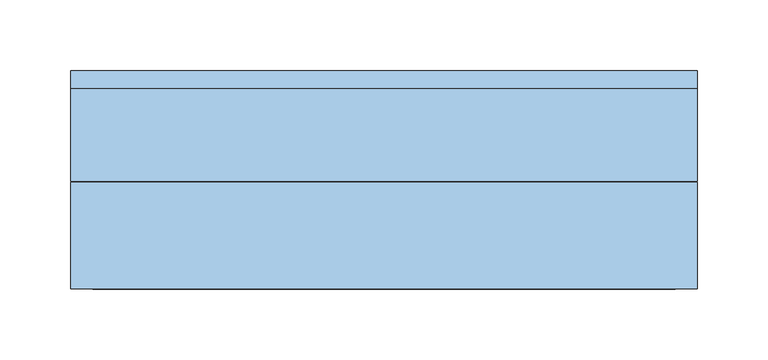
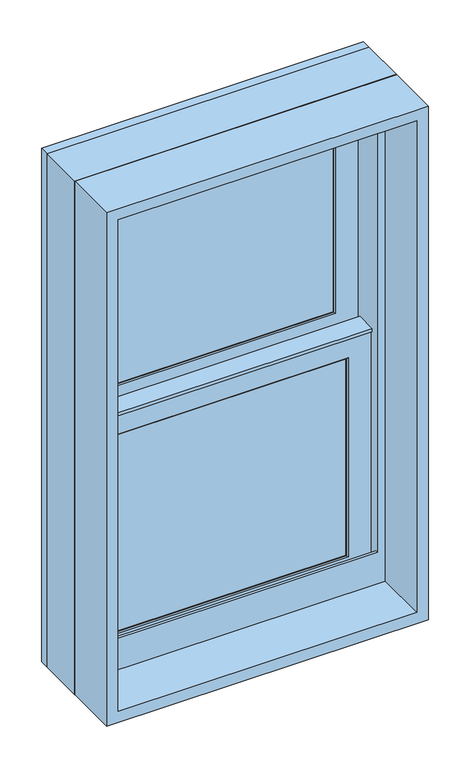
"""IFC4 building model written with IfcOpenShell, lengths in millimetres: window geometry, Window-Double_Hung-Marvin-Essential : ESDH1626."""

from ifc_helpers import new_model, si_unit, frame, origin, place, context, project, spatial, polyline, outline, extrude, faceted_brep, source, transform, mapped, element, save


def window_9d5250ab(model_context):
    return source(origin(), model_context, "Body", "SolidModel", [
        extrude(outline(polyline([(64.5583333, 20.6375), (64.5583333, 15.875), (45.5083333, 15.875), (45.5083333, 20.6375), (64.5583333, 20.6375)])), frame((0.0, 0.0, 1746.25), z_axis=(0.0, 0.0, 1.0), x_axis=(1.0, 0.0, 0.0)), (0.0, 0.0, 1.0), 298.45),
        extrude(outline(polyline([(-45.5083333, 20.6375), (-45.5083333, 15.875), (-64.5583333, 15.875), (-64.5583333, 20.6375), (-45.5083333, 20.6375)])), frame((0.0, 0.0, 1746.25), z_axis=(0.0, 0.0, 1.0), x_axis=(1.0, 0.0, 0.0)), (0.0, 0.0, 1.0), 298.45),
        extrude(outline(polyline([(165.1, 20.6375), (165.1, 15.875), (-165.1, 15.875), (-165.1, 20.6375), (165.1, 20.6375)])), frame((0.0, 0.0, 1885.95), z_axis=(0.0, 0.0, 1.0), x_axis=(1.0, 0.0, 0.0)), (0.0, 0.0, 1.0), 19.05),
        extrude(outline(polyline([(-64.5583333, 46.83125), (-64.5583333, 51.59375), (-45.5083333, 51.59375), (-45.5083333, 46.83125), (-64.5583333, 46.83125)])), frame((0.0, 0.0, 2082.8), z_axis=(0.0, 0.0, 1.0), x_axis=(1.0, 0.0, 0.0)), (0.0, 0.0, 1.0), 298.45),
        extrude(outline(polyline([(45.5083333, 46.83125), (45.5083333, 51.59375), (64.5583333, 51.59375), (64.5583333, 46.83125), (45.5083333, 46.83125)])), frame((0.0, 0.0, 2082.8), z_axis=(0.0, 0.0, 1.0), x_axis=(1.0, 0.0, 0.0)), (0.0, 0.0, 1.0), 298.45),
        extrude(outline(polyline([(-165.1, 46.83125), (-165.1, 51.59375), (165.1, 51.59375), (165.1, 46.83125), (-165.1, 46.83125)])), frame((0.0, 0.0, 2222.5), z_axis=(0.0, 0.0, 1.0), x_axis=(1.0, 0.0, 0.0)), (0.0, 0.0, 1.0), 19.05),
        extrude(outline(polyline([(64.5583333, 20.6375), (45.5083333, 20.6375), (45.5083333, 25.4), (64.5583333, 25.4), (64.5583333, 20.6375)])), frame((0.0, 0.0, 1746.25), z_axis=(0.0, 0.0, 1.0), x_axis=(1.0, 0.0, 0.0)), (0.0, 0.0, 1.0), 298.45),
        extrude(outline(polyline([(-45.5083333, 20.6375), (-64.5583333, 20.6375), (-64.5583333, 25.4), (-45.5083333, 25.4), (-45.5083333, 20.6375)])), frame((0.0, 0.0, 1746.25), z_axis=(0.0, 0.0, 1.0), x_axis=(1.0, 0.0, 0.0)), (0.0, 0.0, 1.0), 298.45),
        extrude(outline(polyline([(165.1, 20.6375), (-165.1, 20.6375), (-165.1, 25.4), (165.1, 25.4), (165.1, 20.6375)])), frame((0.0, 0.0, 1885.95), z_axis=(0.0, 0.0, 1.0), x_axis=(1.0, 0.0, 0.0)), (0.0, 0.0, 1.0), 19.05),
        extrude(outline(polyline([(-64.5583333, 56.35625), (-45.5083333, 56.35625), (-45.5083333, 51.59375), (-64.5583333, 51.59375), (-64.5583333, 56.35625)])), frame((0.0, 0.0, 2082.8), z_axis=(0.0, 0.0, 1.0), x_axis=(1.0, 0.0, 0.0)), (0.0, 0.0, 1.0), 298.45),
        extrude(outline(polyline([(45.5083333, 56.35625), (64.5583333, 56.35625), (64.5583333, 51.59375), (45.5083333, 51.59375), (45.5083333, 56.35625)])), frame((0.0, 0.0, 2082.8), z_axis=(0.0, 0.0, 1.0), x_axis=(1.0, 0.0, 0.0)), (0.0, 0.0, 1.0), 298.45),
        extrude(outline(polyline([(-165.1, 56.35625), (165.1, 56.35625), (165.1, 51.59375), (-165.1, 51.59375), (-165.1, 56.35625)])), frame((0.0, 0.0, 2222.5), z_axis=(0.0, 0.0, 1.0), x_axis=(1.0, 0.0, 0.0)), (0.0, 0.0, 1.0), 19.05),
        faceted_brep([(-192.0875, 5.6780605, 2074.7351748), (-192.0875, 5.6780605, 2070.1), (192.0875, 5.6780605, 2070.1), (192.0875, 5.6780605, 2074.7351748), (-192.0875, 34.8118605, 2074.7351748), (192.0875, 34.8118605, 2074.7351748), (192.0875, 34.8118605, 2070.1), (-192.0875, 34.8118605, 2070.1), (-192.0875, 30.1625, 2070.1), (-192.0875, 30.1625, 1719.2625), (-192.0875, 8.9241104, 1719.2625), (-192.0875, 8.9241104, 2070.1), (192.0875, 8.9241104, 2070.1), (192.0875, 30.1625, 2070.1), (192.0875, 8.9241104, 1719.2625), (192.0875, 30.1625, 1719.2625), (-176.2034752, 11.90625, 2055.8034752), (-176.2034752, 30.1625, 2055.8034752), (176.2034752, 30.1625, 2055.8034752), (176.2034752, 11.90625, 2055.8034752), (-159.54375, 10.4662439, 2039.14375), (-159.54375, 11.90625, 2039.14375), (159.54375, 11.90625, 2039.14375), (159.54375, 10.4662439, 2039.14375), (161.0858834, 8.9241104, 2040.6858834), (-161.0858834, 8.9241104, 2040.6858834), (176.2034752, 30.1625, 1735.1465248), (176.2034752, 11.90625, 1735.1465248), (159.54375, 11.90625, 1751.80625), (159.54375, 10.4662439, 1751.80625), (161.0858834, 8.9241104, 1750.2641166), (-176.2034752, 30.1625, 1735.1465248), (-176.2034752, 11.90625, 1735.1465248), (-159.54375, 11.90625, 1751.80625), (-159.54375, 10.4662439, 1751.80625), (-161.0858834, 8.9241104, 1750.2641166)], [[[0, 1, 2, 3]], [[4, 5, 6, 7]], [[1, 0, 4, 7, 8, 9, 10, 11]], [[2, 1, 11, 12]], [[7, 6, 13, 8]], [[3, 2, 12, 14, 15, 13, 6, 5]], [[0, 3, 5, 4]], [[16, 17, 18, 19]], [[20, 21, 22, 23]], [[20, 23, 24, 25]], [[19, 18, 26, 27]], [[23, 22, 28, 29]], [[24, 23, 29, 30]], [[27, 26, 31, 32]], [[29, 28, 33, 34]], [[30, 29, 34, 35]], [[15, 14, 10, 9]], [[15, 9, 8, 13], [18, 17, 31, 26]], [[17, 16, 32, 31]], [[16, 19, 27, 32], [22, 21, 33, 28]], [[21, 20, 34, 33]], [[20, 25, 35, 34]], [[10, 14, 12, 11], [25, 24, 30, 35]]]),
        extrude(outline(polyline([(38.5955581, 2055.8125), (33.5778968, 2055.8125), (33.5778968, 2057.4), (39.9405976, 2057.4), (39.9405976, 2055.8125), (61.515625, 2055.8125), (47.6307501, 2052.4975159), (38.5955581, 2052.4975159), (38.5955581, 2055.8125)])), frame((-192.0875, 0.0, 0.0), z_axis=(1.0, 0.0, 0.0), x_axis=(0.0, 1.0, 0.0)), (0.0, 0.0, 1.0), 384.175),
        faceted_brep([(222.25, 0.0, 1689.1), (222.25, 0.0, 2438.4), (-222.25, 0.0, 2438.4), (-222.25, 0.0, 1689.1), (196.05625, 0.0, 1750.21875), (-196.05625, 0.0, 1750.21875), (-196.05625, 0.0, 2412.20625), (196.05625, 0.0, 2412.20625), (196.05625, 3.96875, 1689.1), (-196.05625, 3.96875, 1689.1), (-196.05625, 3.96875, 1750.21875), (196.05625, 3.96875, 1750.21875), (-222.25, 65.6828125, 1689.1), (-196.05625, 65.6828125, 1689.1), (196.05625, 65.6828125, 1689.1), (222.25, 65.6828125, 1689.1), (-222.25, 65.6828125, 2438.4), (222.25, 65.6828125, 2438.4), (196.05625, 65.6828125, 2412.20625), (-196.05625, 65.6828125, 2412.20625)], [[[0, 1, 2, 3], [4, 5, 6, 7]], [[8, 9, 10, 11]], [[5, 4, 11, 10]], [[0, 3, 12, 13, 9, 8, 14, 15]], [[13, 12, 16, 17, 15, 14, 18, 19]], [[13, 19, 6, 5, 10, 9]], [[7, 6, 19, 18]], [[18, 14, 8, 11, 4, 7]], [[1, 0, 15, 17]], [[2, 1, 17, 16]], [[3, 2, 16, 12]]]),
        faceted_brep([(196.05625, 30.1625, 2063.75), (194.46875, 30.1625, 2063.75), (194.46875, 30.1625, 1713.4544613), (196.05625, 30.1625, 1713.4544613), (-194.46875, 30.1625, 2063.75), (-196.05625, 30.1625, 2063.75), (-196.05625, 30.1625, 1713.4544613), (-194.46875, 30.1625, 1713.4544613), (194.46875, 63.5, 2063.75), (196.05625, 63.5, 2063.75), (196.05625, 63.5, 1706.9743077), (194.46875, 63.5, 1706.9743077), (-196.05625, 63.5, 2063.75), (-194.46875, 63.5, 2063.75), (-194.46875, 63.5, 1706.9743077), (-196.05625, 63.5, 1706.9743077), (207.3108932, 3.96875, 1718.5460105), (207.3108932, 3.96875, 1689.1), (207.3108932, 65.6828125, 1689.1), (207.3108932, 65.6828125, 1706.550012), (-207.3108932, 3.96875, 1689.1), (-207.3108932, 3.96875, 1718.5460105), (-207.3108932, 65.6828125, 1706.550012), (-207.3108932, 65.6828125, 1689.1), (207.3108932, 78.58125, 1704.0428097), (-207.3108932, 78.58125, 1704.0428097), (-205.2971252, 68.2348864, 1706.0539391), (-187.33135, 68.2348864, 1706.0539391), (-187.33135, 65.6828125, 1706.550012), (187.33135, 65.6828125, 1706.550012), (187.33135, 68.2348864, 1706.0539391), (205.2971252, 68.2348864, 1706.0539391), (-222.25, 65.6828125, 1689.1), (-222.25, 78.5948249, 1689.1), (222.25, 78.5948249, 1689.1), (222.25, 65.6828125, 1689.1), (-222.25, 78.58125, 2438.4), (222.25, 78.58125, 2438.4), (207.3108932, 78.58125, 2423.4608932), (-207.3108932, 78.58125, 2423.4608932), (-222.25, 65.6828125, 2438.4), (-205.2971252, 68.2348864, 2421.4471252), (205.2971252, 68.2348864, 2421.4471252), (187.33135, 68.2348864, 2403.48135), (-187.33135, 68.2348864, 2403.48135), (-187.33135, 65.6828125, 2403.48135), (187.33135, 65.6828125, 2403.48135), (222.25, 65.6828125, 2438.4)], [[[0, 1, 2, 3]], [[4, 5, 6, 7]], [[8, 9, 10, 11]], [[12, 13, 14, 15]], [[1, 8, 11, 2]], [[9, 0, 3, 10]], [[1, 0, 9, 8]], [[5, 4, 13, 12]], [[5, 12, 15, 6]], [[13, 4, 7, 14]], [[16, 17, 18, 19]], [[20, 21, 22, 23]], [[24, 25, 26, 27, 28, 22, 21, 16, 19, 29, 30, 31], [3, 2, 11, 10], [7, 6, 15, 14]], [[17, 16, 21, 20]], [[17, 20, 23, 32, 33, 34, 35, 18]], [[34, 33, 36, 37], [25, 24, 38, 39]], [[33, 32, 40, 36]], [[39, 41, 26, 25]], [[41, 42, 31, 30, 43, 44, 27, 26]], [[44, 45, 28, 27]], [[40, 32, 23, 22, 28, 45, 46, 29, 19, 18, 35, 47]], [[36, 40, 47, 37]], [[39, 38, 42, 41]], [[44, 43, 46, 45]], [[34, 37, 47, 35]], [[42, 38, 24, 31]], [[46, 43, 30, 29]]]),
        extrude(outline(polyline([(172.24375, 11.90625), (-172.24375, 11.90625), (-172.24375, 15.08125), (172.24375, 15.08125), (172.24375, 11.90625)])), frame((0.0, 0.0, 1739.10625), z_axis=(0.0, 0.0, 1.0), x_axis=(1.0, 0.0, 0.0)), (0.0, 0.0, 1.0), 312.7375),
        extrude(outline(polyline([(172.24375, 42.8625), (-172.24375, 42.8625), (-172.24375, 46.0375), (172.24375, 46.0375), (172.24375, 42.8625)])), frame((0.0, 0.0, 2075.65625), z_axis=(0.0, 0.0, 1.0), x_axis=(1.0, 0.0, 0.0)), (0.0, 0.0, 1.0), 312.7375),
        faceted_brep([(-159.54375, 31.194477, 2039.14375), (-161.0858834, 32.7366104, 2040.6858834), (161.0858834, 32.7366104, 2040.6858834), (159.54375, 31.194477, 2039.14375), (-159.54375, 30.1625, 2039.14375), (159.54375, 30.1625, 2039.14375), (-192.0875, 32.7366104, 2071.6875), (-192.0875, 30.1625, 2071.6875), (192.0875, 30.1625, 2071.6875), (192.0875, 32.7366104, 2071.6875), (161.0858834, 32.7366104, 1750.2641166), (159.54375, 31.194477, 1751.80625), (159.54375, 30.1625, 1751.80625), (192.0875, 30.1625, 1719.2625), (192.0875, 32.7366104, 1719.2625), (-161.0858834, 32.7366104, 1750.2641166), (-159.54375, 31.194477, 1751.80625), (-159.54375, 30.1625, 1751.80625), (-192.0875, 30.1625, 1719.2625), (-192.0875, 32.7366104, 1719.2625)], [[[0, 1, 2, 3]], [[4, 0, 3, 5]], [[6, 7, 8, 9]], [[3, 2, 10, 11]], [[5, 3, 11, 12]], [[9, 8, 13, 14]], [[11, 10, 15, 16]], [[12, 11, 16, 17]], [[14, 13, 18, 19]], [[9, 14, 19, 6], [1, 15, 10, 2]], [[16, 15, 1, 0]], [[17, 16, 0, 4]], [[7, 18, 13, 8], [5, 12, 17, 4]], [[19, 18, 7, 6]]]),
        faceted_brep([(-176.2034752, 42.8625, 2392.3534752), (-176.2034752, 61.11875, 2392.3534752), (176.2034752, 61.11875, 2392.3534752), (176.2034752, 42.8625, 2392.3534752), (-159.54375, 41.4224939, 2375.69375), (-159.54375, 42.8625, 2375.69375), (159.54375, 42.8625, 2375.69375), (159.54375, 41.4224939, 2375.69375), (-161.0858834, 39.8803604, 2377.2358834), (161.0858834, 39.8803604, 2377.2358834), (-192.0875, 61.11875, 2408.2375), (-192.0875, 39.8803604, 2408.2375), (192.0875, 39.8803604, 2408.2375), (192.0875, 61.11875, 2408.2375), (176.2034752, 61.11875, 2071.6965248), (176.2034752, 42.8625, 2071.6965248), (159.54375, 42.8625, 2088.35625), (159.54375, 41.4224939, 2088.35625), (161.0858834, 39.8803604, 2086.8141166), (192.0875, 39.8803604, 2055.8125), (192.0875, 61.11875, 2055.8125), (-176.2034752, 61.11875, 2071.6965248), (-176.2034752, 42.8625, 2071.6965248), (-159.54375, 42.8625, 2088.35625), (-159.54375, 41.4224939, 2088.35625), (-161.0858834, 39.8803604, 2086.8141166), (-192.0875, 39.8803604, 2055.8125), (-192.0875, 61.11875, 2055.8125)], [[[0, 1, 2, 3]], [[4, 5, 6, 7]], [[8, 4, 7, 9]], [[10, 11, 12, 13]], [[3, 2, 14, 15]], [[7, 6, 16, 17]], [[9, 7, 17, 18]], [[13, 12, 19, 20]], [[15, 14, 21, 22]], [[17, 16, 23, 24]], [[18, 17, 24, 25]], [[20, 19, 26, 27]], [[13, 20, 27, 10], [1, 21, 14, 2]], [[22, 21, 1, 0]], [[3, 15, 22, 0], [5, 23, 16, 6]], [[24, 23, 5, 4]], [[25, 24, 4, 8]], [[11, 26, 19, 12], [9, 18, 25, 8]], [[27, 26, 11, 10]]]),
        faceted_brep([(-192.0875, 61.11875, 2055.8125), (-192.0875, 63.6928604, 2055.8125), (192.0875, 63.6928604, 2055.8125), (192.0875, 61.11875, 2055.8125), (-159.54375, 62.150727, 2088.35625), (-159.54375, 61.11875, 2088.35625), (159.54375, 61.11875, 2088.35625), (159.54375, 62.150727, 2088.35625), (-161.0858834, 63.6928604, 2086.8141166), (161.0858834, 63.6928604, 2086.8141166), (192.0875, 63.6928604, 2408.2375), (192.0875, 61.11875, 2408.2375), (159.54375, 61.11875, 2375.69375), (159.54375, 62.150727, 2375.69375), (161.0858834, 63.6928604, 2377.2358834), (-192.0875, 63.6928604, 2408.2375), (-192.0875, 61.11875, 2408.2375), (-159.54375, 61.11875, 2375.69375), (-159.54375, 62.150727, 2375.69375), (-161.0858834, 63.6928604, 2377.2358834)], [[[0, 1, 2, 3]], [[4, 5, 6, 7]], [[8, 4, 7, 9]], [[3, 2, 10, 11]], [[7, 6, 12, 13]], [[9, 7, 13, 14]], [[11, 10, 15, 16]], [[13, 12, 17, 18]], [[14, 13, 18, 19]], [[16, 15, 1, 0]], [[3, 11, 16, 0], [5, 17, 12, 6]], [[18, 17, 5, 4]], [[19, 18, 4, 8]], [[1, 15, 10, 2], [9, 14, 19, 8]]]),
        extrude(outline(polyline([(172.24375, 26.19375), (-172.24375, 26.19375), (-172.24375, 30.1625), (172.24375, 30.1625), (172.24375, 26.19375)])), frame((0.0, 0.0, 1739.10625), z_axis=(0.0, 0.0, 1.0), x_axis=(1.0, 0.0, 0.0)), (0.0, 0.0, 1.0), 312.7375),
        extrude(outline(polyline([(172.24375, 57.15), (-172.24375, 57.15), (-172.24375, 61.11875), (172.24375, 61.11875), (172.24375, 57.15)])), frame((0.0, 0.0, 2075.65625), z_axis=(0.0, 0.0, 1.0), x_axis=(1.0, 0.0, 0.0)), (0.0, 0.0, 1.0), 312.7375),
        extrude(outline(polyline([(2438.4, 222.25), (2438.4, -222.25), (1689.1, -222.25), (1689.1, 222.25), (2438.4, 222.25)]), holes=[polyline([(2422.525, 206.375), (1704.975, 206.375), (1704.975, -206.375), (2422.525, -206.375), (2422.525, 206.375)])]), frame((0.0, -76.2, 0.0), z_axis=(0.0, 1.0, 0.0), x_axis=(0.0, 0.0, 1.0)), (0.0, 0.0, 1.0), 75.40625),
    ])


if __name__ == "__main__":
    model = new_model("IFC4")
    model_context = context("Model", 3, world=origin())
    ifc_project = project(units=[si_unit("LENGTHUNIT", "METRE", prefix="MILLI")], contexts=[model_context])
    site = spatial("IfcSite", under=ifc_project)
    building = spatial("IfcBuilding", under=site)
    placement = place(None, origin())
    window_shape = window_9d5250ab(model_context)
    element("IfcWindow", 1, ObjectType="Window-Double_Hung-Marvin-Essential : ESDH1626", at=placement, inside=building, context=model_context, shape_type="MappedRepresentation", body=[
        mapped(window_shape, transform((0.0, 0.0, 0.0), x_axis=(1.0, 0.0, 0.0), y_axis=(0.0, 1.0, 0.0), z_axis=(0.0, 0.0, 1.0))),
    ])
    save(model, "model.ifc")

# Revit data of these elements
# Type "Window-Double_Hung-Marvin-Essential : ESDH1626"
#   Type Mark = "26"
#   Window Type = "Essential Double Hung"
#   Product data url = "https://bimobject.com/marvin-windows-and-doors/product/marvin-dhwau"
#   Product Guid = "c4a96547-874c-4385-91dc-a058adc19d98"
#   Frame = "All Ultrex"
#   Egress Window = "No"
#   URL = "www.marvin.com"
#   Model = "ESDH1626"
#   Manufacturer = "Marvin Windows and Doors"
#   Label Egress = ""
#   Glass Type = "IG Low E II with Argon"
#   Design Pressure = "DP50"
#   Description = "1830 DBHG"
#   Analytic Construction = "<None>"
#   Prairie Corner Width = 0' - 4"
#   Prairie Corner Height = 0' - 4"
#   Egress Width = 1' - 2 9/16"
#   Egress Height = 0' - 10 27/128"
#   Rough Width = 1' - 6"
#   Rough Height = 2' - 6"
#   Nominal Width = 1' - 6"
#   Nominal Height = 2' - 6"
#   Inset to Installation Flange [instance default] = 0' - 1"
#   Height = 2' - 5 1/2"
#   Egress Area = 1.03262 SF
#   Default Head Height = 8' - 0"
#   Width = 1' - 5 1/2"
#   Daylight Area = 1.9738 SF
#   DLO Width = 1' - 0 9/16"
#   DLO Height = 0' - 11 5/16"
#   Muntins Top Sash = yes
#   Lites Wide Top Sash = 3
#   Lites Wide Bottom Sash = 3
#   Lites High Top Sash = 2
#   Lites High Bottom Sash = 2
#   Lite Cut Prairie 9 = no
#   Lite Cut HV Grid = yes
#   Muntins Bottom Sash = yes
#   Label Visibility = no
#   Jamb Extension Visibility = yes
#   Edition number = 1
#   Interior Material = Ultrex-Marvin-Stonewhite
#   Glazing Material = Glass-Marvin-IG Low E II with Argon
#   Cladding Material = Ultrex-Marvin-Pebblegray
#   Wall Closure = (empty or 0)
#   Assembly Code = ""
# Element 1 (IfcWindow, "Window-Double_Hung-Marvin-Essential : ESDH1626")
#   Materials on its faces: "Ultrex-Marvin-Pebblegray", "Ultrex-Marvin-Stonewhite", "Glass-Marvin-IG Low E II with Argon"
# Materials
#   "Ultrex-Marvin-Stonewhite": class "Paint", colour RGB 250 251 245, transparency 0
#   "Glass-Marvin-IG Low E II with Argon": class "Glass", colour RGB 0 128 192, transparency 0.85
#   "Ultrex-Marvin-Pebblegray": class "Paint", colour RGB 189 185 173, transparency 0
